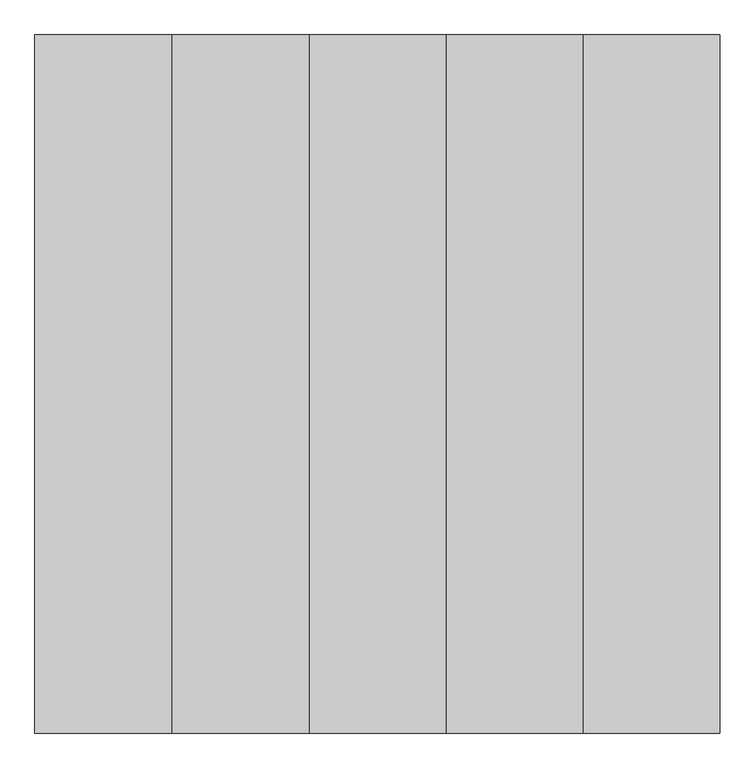
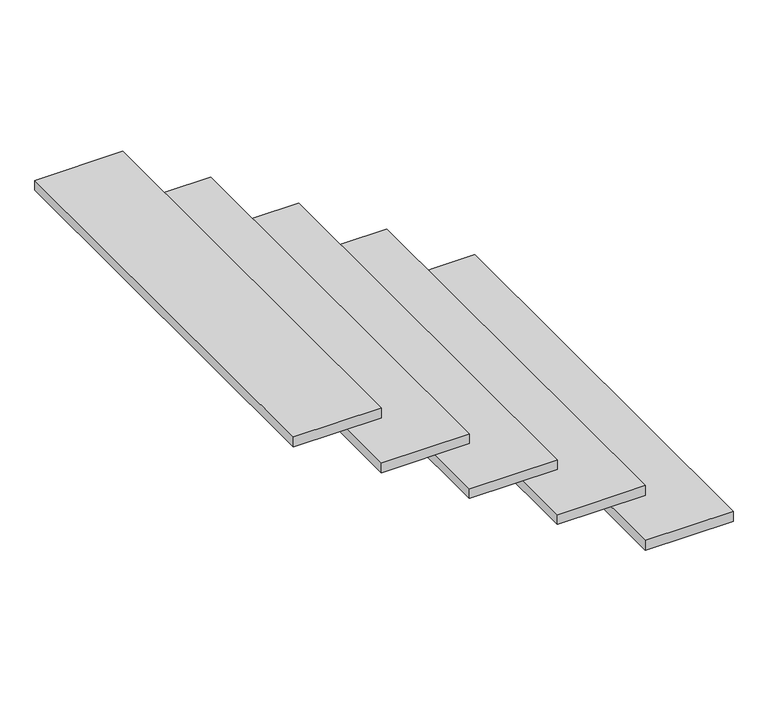
"""IFC4 building model written with IfcOpenShell, lengths in millimetres: stair flight geometry."""

import ifcopenshell
import ifcopenshell.guid

model = None  # the IFC model being written
_history = None  # IfcOwnerHistory: only IFC2X3 demands one
_inside = {}  # id of a spatial element -> (the spatial element, [elements in it])
_under = {}  # id of a project, library or spatial element -> (it, [spatial elements below it])
_declared = {}  # id of a project -> (the project, [libraries it declares])
_typed = {}  # id of a type object -> (the type object, [elements of that type])
_made_of = {}  # id of a material, layer set ... -> (it, [elements and type objects made of it])


def new_model(schema):
    """Start an empty IFC model of exactly this schema.

    Asked for "IFC4X3", IfcOpenShell would pick the latest addendum, in which some entities
    have other attributes; the version numbers below select the first issue.
    IFC2X3 requires an IfcOwnerHistory on every rooted entity: one is made here for all.
    """
    global model, _history
    if schema == "IFC4X3":
        model = ifcopenshell.file(schema_version=(4, 3, 0, 0))
    else:
        model = ifcopenshell.file(schema=schema)
    _inside.clear()
    _under.clear()
    _declared.clear()
    _typed.clear()
    _made_of.clear()
    _history = None
    if model.schema == "IFC2X3":
        org = make("IfcOrganization", Name="unknown")
        user = make(
            "IfcPersonAndOrganization",
            ThePerson=make("IfcPerson", FamilyName="unknown"),
            TheOrganization=org,
        )
        app = make(
            "IfcApplication",
            ApplicationDeveloper=org,
            Version="unknown",
            ApplicationFullName="unknown",
            ApplicationIdentifier="unknown",
        )
        _history = make(
            "IfcOwnerHistory",
            OwningUser=user,
            OwningApplication=app,
            ChangeAction="ADDED",
            CreationDate=0,
        )
    return model


def make(cls, **values):
    """One entity of the class cls with the attributes given. An attribute that is None is left unset."""
    return model.create_entity(
        cls, **{name: value for name, value in values.items() if value is not None}
    )


def rooted(cls, **values):
    """An entity with a GlobalId (a new one), such as an element, a storey or a relation."""
    return make(cls, GlobalId=ifcopenshell.guid.new(), OwnerHistory=_history, **values)


def si_unit(unit_type, name, prefix=None):
    """IfcSIUnit, for example si_unit("LENGTHUNIT", "METRE", prefix="MILLI")."""
    return make("IfcSIUnit", UnitType=unit_type, Prefix=prefix, Name=name)


def assignment(units):
    """IfcUnitAssignment: the units of a project."""
    return None if units is None else make("IfcUnitAssignment", Units=units)


def point(xyz):
    """IfcCartesianPoint."""
    return None if xyz is None else make("IfcCartesianPoint", Coordinates=xyz)


def direction(xyz):
    """IfcDirection."""
    return None if xyz is None else make("IfcDirection", DirectionRatios=xyz)


def frame(location, z_axis=None, x_axis=None):
    """IfcAxis2Placement3D, a coordinate frame: its origin and axes. An axis left out is left unset."""
    return make(
        "IfcAxis2Placement3D",
        Location=point(location),
        Axis=direction(z_axis),
        RefDirection=direction(x_axis),
    )


def origin():
    """The frame at (0, 0, 0) with its axes left unset."""
    return frame((0.0, 0.0, 0.0))


def place(relative_to, where):
    """IfcLocalPlacement: puts the frame where relative to a parent placement (None: the world)."""
    return make(
        "IfcLocalPlacement", PlacementRelTo=relative_to, RelativePlacement=where
    )


def context(
    kind, dimensions, precision=None, world=None, true_north=None, identifier=None
):
    """IfcGeometricRepresentationContext, for example the 3D "Model" context."""
    return make(
        "IfcGeometricRepresentationContext",
        ContextIdentifier=identifier,
        ContextType=kind,
        CoordinateSpaceDimension=dimensions,
        Precision=precision,
        WorldCoordinateSystem=world,
        TrueNorth=true_north,
    )


def project(units=None, contexts=None):
    """IfcProject with its units and contexts."""
    return rooted(
        "IfcProject",
        Name="project",
        RepresentationContexts=contexts,
        UnitsInContext=assignment(units),
    )


def spatial(cls, under=None, at=None, **own):
    """A site, building, storey or space (cls), placed at a placement, below another one or the project."""
    s = rooted(cls, ObjectPlacement=at, **own)
    if under is not None:
        _under.setdefault(under.id(), (under, []))[1].append(s)
    return s


def polyline(points):
    """IfcPolyline through the points."""
    return make("IfcPolyline", Points=[point(p) for p in points])


def outline(outer, holes=None, kind="AREA"):
    """IfcArbitraryClosedProfileDef: a profile drawn as a closed curve; with holes, ...WithVoids."""
    if holes is None:
        return make("IfcArbitraryClosedProfileDef", ProfileType=kind, OuterCurve=outer)
    return make(
        "IfcArbitraryProfileDefWithVoids",
        ProfileType=kind,
        OuterCurve=outer,
        InnerCurves=holes,
    )


def extrude(swept, where, along, depth):
    """IfcExtrudedAreaSolid: the profile swept, set in the frame where, extruded along a direction by depth."""
    return make(
        "IfcExtrudedAreaSolid",
        SweptArea=swept,
        Position=where,
        ExtrudedDirection=direction(along),
        Depth=depth,
    )


def shape(context_of_items, identifier, shape_type, items):
    """IfcShapeRepresentation: the items that make up one representation, for example the "Body"."""
    return make(
        "IfcShapeRepresentation",
        ContextOfItems=context_of_items,
        RepresentationIdentifier=identifier,
        RepresentationType=shape_type,
        Items=items,
    )


def source(mapping_origin, context_of_items, identifier, shape_type, items):
    """IfcRepresentationMap: a shape defined once, which mapped items show again and again."""
    return make(
        "IfcRepresentationMap",
        MappingOrigin=mapping_origin,
        MappedRepresentation=shape(context_of_items, identifier, shape_type, items),
    )


def transform(
    local_origin,
    x_axis=None,
    y_axis=None,
    z_axis=None,
    scale=None,
    scale2=None,
    scale3=None,
    uniform=True,
):
    """IfcCartesianTransformationOperator3D, or its non-uniform kind. x_axis, y_axis, z_axis: its Axis1, 2, 3."""
    if uniform:
        return make(
            "IfcCartesianTransformationOperator3D",
            Axis1=direction(x_axis),
            Axis2=direction(y_axis),
            LocalOrigin=point(local_origin),
            Scale=scale,
            Axis3=direction(z_axis),
        )
    return make(
        "IfcCartesianTransformationOperator3DnonUniform",
        Axis1=direction(x_axis),
        Axis2=direction(y_axis),
        LocalOrigin=point(local_origin),
        Scale=scale,
        Axis3=direction(z_axis),
        Scale2=scale2,
        Scale3=scale3,
    )


def mapped(mapping_source, mapping_target):
    """IfcMappedItem: shows the shape of a source again, moved by a transform."""
    return make(
        "IfcMappedItem", MappingSource=mapping_source, MappingTarget=mapping_target
    )


def made_of(thing, what):
    """Note that an element or type object is made of a material, layer set ...; save() writes the relation."""
    if what is not None:
        _made_of.setdefault(what.id(), (what, []))[1].append(thing)
    return thing


def element(
    cls,
    number,
    at=None,
    inside=None,
    cuts=None,
    type_object=None,
    material=None,
    context=None,
    identifier="Body",
    shape_type=None,
    held_by="IfcProductDefinitionShape",
    body=None,
    shapes=None,
    **own,
):
    """One element of the class cls, such as IfcWall. Its Tag is "e" and its number.

    at: its placement. inside: the storey or other place that contains it. cuts: it is an
    opening in that element (IfcRelVoidsElement). A single representation is given by context,
    identifier, shape_type and body (its items); several are given by shapes. held_by: the class
    of the entity that holds the representations. save() writes the other relations.
    """
    e = rooted(cls, Tag="e%d" % number, ObjectPlacement=at, **own)
    if body is not None:
        shapes = [shape(context, identifier, shape_type, body)]
    if shapes is not None:
        e.Representation = make(held_by, Representations=shapes)
    if inside is not None:
        _inside.setdefault(inside.id(), (inside, []))[1].append(e)
    if cuts is not None:
        rooted(
            "IfcRelVoidsElement", RelatingBuildingElement=cuts, RelatedOpeningElement=e
        )
    if type_object is not None:
        _typed.setdefault(type_object.id(), (type_object, []))[1].append(e)
    return made_of(e, material)


def aggregate(whole, parts):
    """IfcRelAggregates: a whole, such as a stair, and the parts it consists of."""
    return rooted("IfcRelAggregates", RelatingObject=whole, RelatedObjects=parts)


def save(model, path):
    """Write the relations noted so far, then the file.

    IfcRelAggregates (storeys below a building ...), IfcRelContainedInSpatialStructure (elements
    in a storey), IfcRelDefinesByType, IfcRelAssociatesMaterial and IfcRelDeclares: one each for
    every whole, place, type object, material and project.
    """
    for whole, parts in _under.values():
        aggregate(whole, parts)
    for where, things in _inside.values():
        rooted(
            "IfcRelContainedInSpatialStructure",
            RelatedElements=things,
            RelatingStructure=where,
        )
    for kind, things in _typed.values():
        rooted("IfcRelDefinesByType", RelatedObjects=things, RelatingType=kind)
    for what, things in _made_of.values():
        rooted("IfcRelAssociatesMaterial", RelatedObjects=things, RelatingMaterial=what)
    for by, libraries in _declared.values():
        rooted("IfcRelDeclares", RelatingContext=by, RelatedDefinitions=libraries)
    model.write(path)


def stair_flight_4e27faa5(model_context):
    return source(origin(), model_context, "Body", "SweptSolid", [
        extrude(outline(polyline([(47808.2332408, 6860.0306666), (47808.2332408, 8235.0306666), (48078.2332408, 8235.0306666), (48078.2332408, 6860.0306666), (47808.2332408, 6860.0306666)])), frame((0.0, 0.0, 296.5714286), z_axis=(0.0, 0.0, 1.0), x_axis=(1.0, 0.0, 0.0)), (0.0, 0.0, 1.0), 32.0),
        extrude(outline(polyline([(47538.2332408, 6860.0306666), (47538.2332408, 8235.0306666), (47808.2332408, 8235.0306666), (47808.2332408, 6860.0306666), (47538.2332408, 6860.0306666)])), frame((0.0, 0.0, 475.1428571), z_axis=(0.0, 0.0, 1.0), x_axis=(1.0, 0.0, 0.0)), (0.0, 0.0, 1.0), 32.0),
        extrude(outline(polyline([(47268.2332408, 6860.0306666), (47268.2332408, 8235.0306666), (47538.2332408, 8235.0306666), (47538.2332408, 6860.0306666), (47268.2332408, 6860.0306666)])), frame((0.0, 0.0, 653.7142857), z_axis=(0.0, 0.0, 1.0), x_axis=(1.0, 0.0, 0.0)), (0.0, 0.0, 1.0), 32.0),
        extrude(outline(polyline([(46998.2332408, 6860.0306666), (46998.2332408, 8235.0306666), (47268.2332408, 8235.0306666), (47268.2332408, 6860.0306666), (46998.2332408, 6860.0306666)])), frame((0.0, 0.0, 832.2857143), z_axis=(0.0, 0.0, 1.0), x_axis=(1.0, 0.0, 0.0)), (0.0, 0.0, 1.0), 32.0),
        extrude(outline(polyline([(46728.2332408, 6860.0306666), (46728.2332408, 8235.0306666), (46998.2332408, 8235.0306666), (46998.2332408, 6860.0306666), (46728.2332408, 6860.0306666)])), frame((0.0, 0.0, 1010.8571429), z_axis=(0.0, 0.0, 1.0), x_axis=(1.0, 0.0, 0.0)), (0.0, 0.0, 1.0), 32.0),
    ])


if __name__ == "__main__":
    model = new_model("IFC4")
    model_context = context("Model", 3, world=origin())
    ifc_project = project(units=[si_unit("LENGTHUNIT", "METRE", prefix="MILLI")], contexts=[model_context])
    site = spatial("IfcSite", under=ifc_project)
    building = spatial("IfcBuilding", under=site)
    placement = place(None, origin())
    stair_flight_shape = stair_flight_4e27faa5(model_context)
    element("IfcStairFlight", 1, at=placement, inside=building, context=model_context, shape_type="MappedRepresentation", body=[
        mapped(stair_flight_shape, transform((0.0, 0.0, 0.0), x_axis=(1.0, 0.0, 0.0), y_axis=(0.0, 1.0, 0.0), z_axis=(0.0, 0.0, 1.0))),
    ])
    save(model, "model.ifc")
